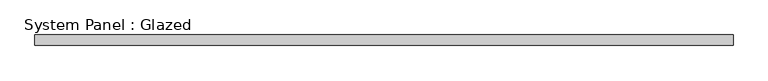
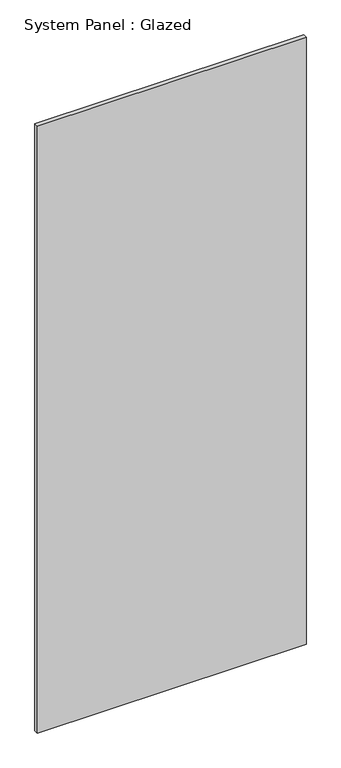
"""IFC4 building model written with IfcOpenShell, lengths in millimetres: plate geometry, System Panel : Glazed."""

from ifc_helpers import new_model, si_unit, origin, origin_with_axes, place, context, project, spatial, polyline, outline, extrude, source, transform, mapped, element, save


def system_panel_glazed_d2268581(model_context):
    return source(origin(), model_context, "Body", "SweptSolid", [
        extrude(outline(polyline([(827.5000002, 24.5), (-827.5000002, 24.5), (-827.5000002, 49.5), (827.5000002, 49.5), (827.5000002, 24.5)])), origin_with_axes(), (0.0, 0.0, 1.0), 3950.0),
    ])


if __name__ == "__main__":
    model = new_model("IFC4")
    model_context = context("Model", 3, world=origin())
    ifc_project = project(units=[si_unit("LENGTHUNIT", "METRE", prefix="MILLI")], contexts=[model_context])
    site = spatial("IfcSite", under=ifc_project)
    building = spatial("IfcBuilding", under=site)
    placement = place(None, origin())
    system_panel_glazed_shape = system_panel_glazed_d2268581(model_context)
    element("IfcPlate", 1, ObjectType="System Panel : Glazed", at=placement, inside=building, context=model_context, shape_type="MappedRepresentation", body=[
        mapped(system_panel_glazed_shape, transform((0.0, 0.0, 0.0), x_axis=(1.0, 0.0, 0.0), y_axis=(0.0, 1.0, 0.0), z_axis=(0.0, 0.0, 1.0))),
    ])
    save(model, "model.ifc")

# Revit data of these elements
# Type "System Panel : Glazed"
#   Keynote = "H11"
#   Construction Type Id = "GSP4R"
#   Analytic Construction = "1/8 in Pilkington single glazing"
#   Visual Light Transmittance = 0.9
#   Solar Heat Gain Coefficient = 0.86
#   Heat Transfer Coefficient (U) = 6.7069 W/(m²·K)
#   Define Thermal Properties by = 1
# Element 1 (IfcPlate, "System Panel : Glazed")
#   Materials on its faces: "Glass"
# Materials
#   "Glass": class "Glass", colour RGB 0 128 192, transparency 0.9, Description = "Soda Lime Glass", Cost = 0
